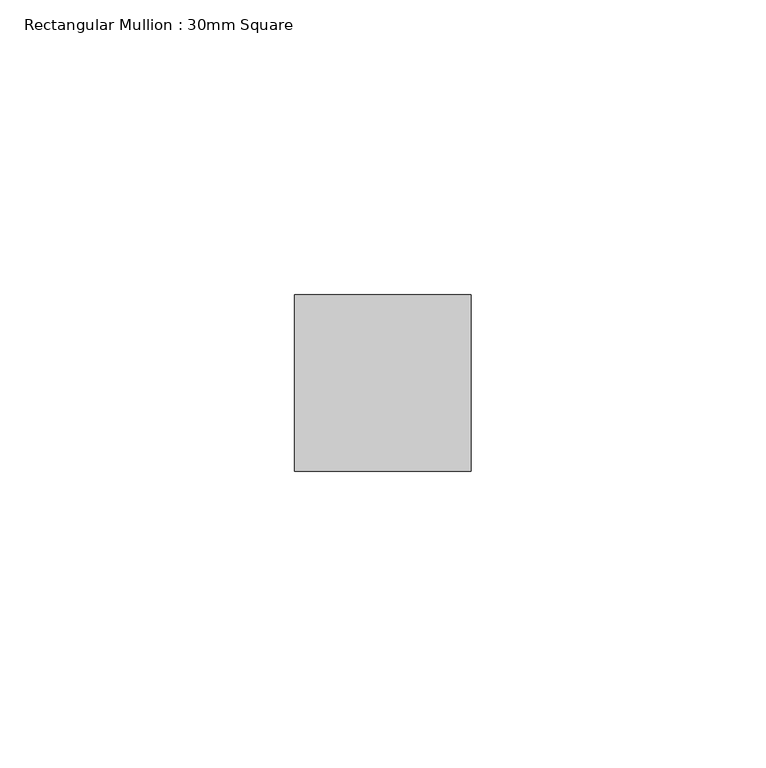
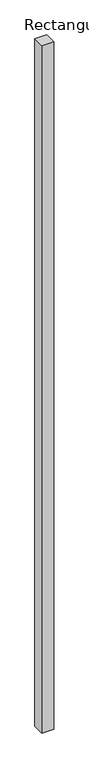
"""IFC4 building model written with IfcOpenShell, lengths in millimetres: member geometry, Rectangular Mullion : 30mm Square."""

from ifc_helpers import new_model, si_unit, frame, origin, place, context, project, spatial, polyline, outline, extrude, source, transform, mapped, element, save


def rectangular_mullion_30mm_square_8e68c213(model_context):
    return source(origin(), model_context, "Body", "SweptSolid", [
        extrude(outline(polyline([(15.0, 15.0), (15.0, -15.0), (-15.0, -15.0), (-15.0, 15.0), (15.0, 15.0)])), frame((0.0, 0.0, -1840.2360175), z_axis=(0.0, 0.0, 1.0), x_axis=(1.0, 0.0, 0.0)), (0.0, 0.0, 1.0), 1840.2360175),
    ])


if __name__ == "__main__":
    model = new_model("IFC4")
    model_context = context("Model", 3, world=origin())
    ifc_project = project(units=[si_unit("LENGTHUNIT", "METRE", prefix="MILLI")], contexts=[model_context])
    site = spatial("IfcSite", under=ifc_project)
    building = spatial("IfcBuilding", under=site)
    placement = place(None, origin())
    rectangular_mullion_30mm_square_shape = rectangular_mullion_30mm_square_8e68c213(model_context)
    element("IfcMember", 1, ObjectType="Rectangular Mullion : 30mm Square", at=placement, inside=building, context=model_context, shape_type="MappedRepresentation", body=[
        mapped(rectangular_mullion_30mm_square_shape, transform((0.0, 0.0, 0.0), x_axis=(1.0, 0.0, 0.0), y_axis=(0.0, 1.0, 0.0), z_axis=(0.0, 0.0, 1.0))),
    ])
    save(model, "model.ifc")

# Revit data of these elements
# Type "Rectangular Mullion : 30mm Square"
#   built-in parameter 1007304 = 0.0984252 (stored number, unit not read)
#   built-in parameter 1007301 = 0.0492126 (stored number, unit not read)
#   built-in parameter 1007300 = 0.0492126 (stored number, unit not read)
# Element 1 (IfcMember, "Rectangular Mullion : 30mm Square")
#   Materials on its faces: "Aluminum"
# Materials
#   "Aluminum": class "Metal", colour RGB 244 244 244, transparency 0, Description = "Aluminum 6061", Cost = 0
